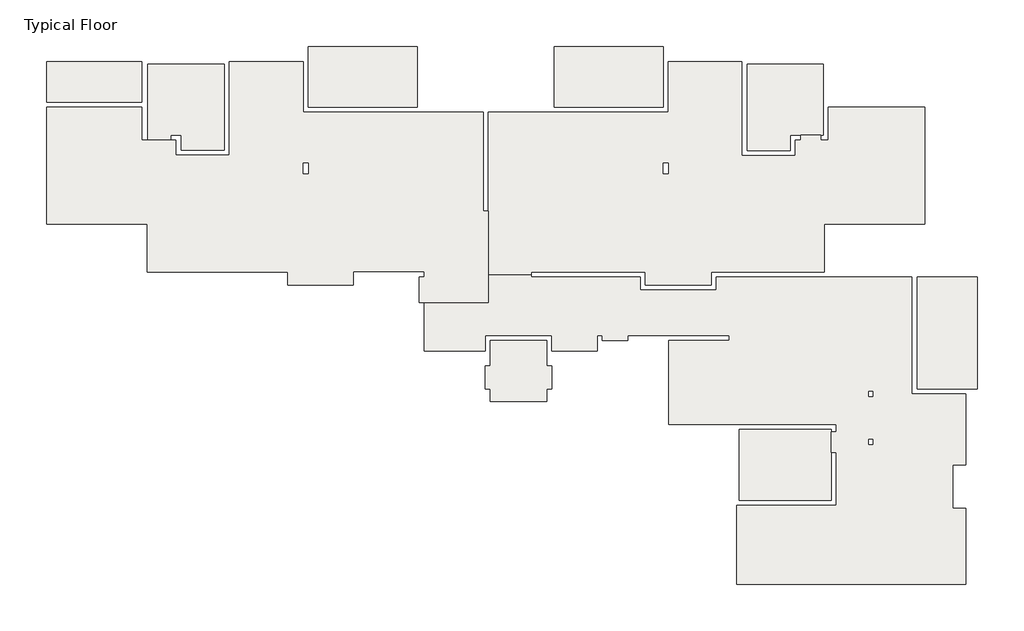
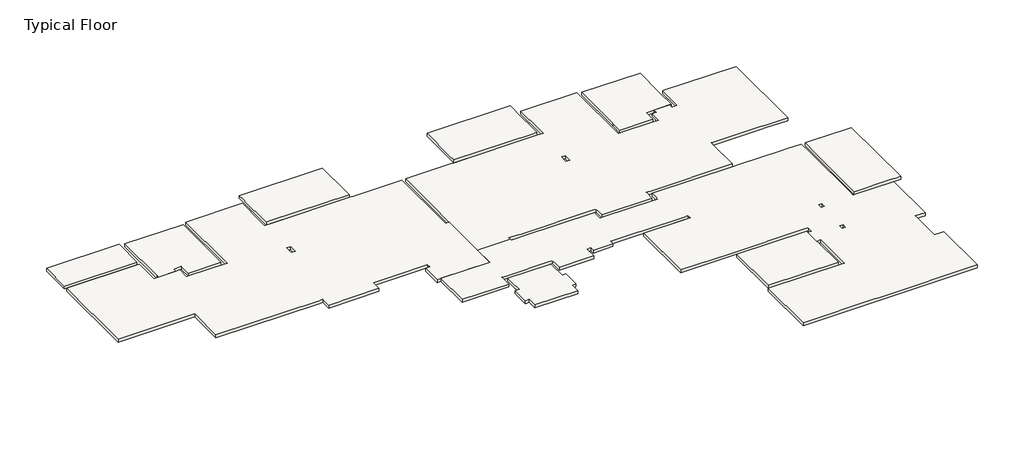
# One storey: 11 slabs.
"""IFC4 building model written with IfcOpenShell, lengths in millimetres."""

from ifc_helpers import new_model, si_unit, origin, place, context, project, spatial, faceted_brep, element, save

model = new_model("IFC4")

# Units and contexts
model_context = context("Model", 3, world=origin())
ifc_project = project(units=[si_unit("LENGTHUNIT", "METRE", prefix="MILLI")], contexts=[model_context])

# Site, building, storey
site = spatial("IfcSite", under=ifc_project)
building = spatial("IfcBuilding", under=site)
storey = spatial("IfcBuildingStorey", under=building, Name="Typical Floor", Elevation=3000.0)

# Slabs
placement = place(None, origin())
element("IfcSlab", 1, ObjectType="16", at=placement, inside=storey, context=model_context, shape_type="Brep", body=[
    faceted_brep([(21265.0782187, -24925.0312743, 2840.0), (21465.0782187, -24925.0312743, 2840.0), (21465.0782187, -24325.0312743, 2840.0), (21465.0782187, -23922.9713632, 2840.0), (23683.1266142, -23922.9713632, 2840.0), (23683.1266142, -24325.0312743, 2840.0), (23683.1266142, -24525.0312743, 2840.0), (23683.1266142, -24925.0312743, 2840.0), (23883.1266142, -24925.0312743, 2840.0), (23883.1266142, -25822.9713632, 2840.0), (23683.1266142, -25822.9713632, 2840.0), (23683.1266142, -26322.9713632, 2840.0), (21465.0782187, -26322.9713632, 2840.0), (21465.0782187, -25822.9713632, 2840.0), (21265.0782187, -25822.9713632, 2840.0), (21465.0782187, -24925.0312743, 3000.0), (21265.0782187, -24925.0312743, 3000.0), (21265.0782187, -25822.9713632, 3000.0), (21465.0782187, -25822.9713632, 3000.0), (21465.0782187, -26322.9713632, 3000.0), (23683.1266142, -26322.9713632, 3000.0), (23683.1266142, -25822.9713632, 3000.0), (23883.1266142, -25822.9713632, 3000.0), (23883.1266142, -24925.0312743, 3000.0), (23683.1266142, -24925.0312743, 3000.0), (23683.1266142, -24525.0312743, 3000.0), (23683.1266142, -24325.0312743, 3000.0), (23683.1266142, -23922.9713632, 3000.0), (21465.0782187, -23922.9713632, 3000.0), (21465.0782187, -24325.0312743, 3000.0), (23683.1266142, -26322.9713632, 2850.0), (21465.0782187, -26322.9713632, 2850.0)], [[[0, 1, 2, 3, 4, 5, 6, 7, 8, 9, 10, 11, 12, 13, 14]], [[15, 16, 17, 18, 19, 20, 21, 22, 23, 24, 25, 26, 27, 28, 29]], [[1, 0, 16, 15]], [[1, 15, 29, 28, 3, 2]], [[4, 3, 28, 27]], [[4, 27, 26, 25, 24, 7, 6, 5]], [[8, 7, 24, 23]], [[9, 8, 23, 22]], [[10, 9, 22, 21]], [[11, 10, 21, 20, 30]], [[12, 11, 30, 20, 19, 31]], [[13, 12, 31, 19, 18]], [[14, 13, 18, 17]], [[0, 14, 17, 16]]]),
])
element("IfcSlab", 2, ObjectType="16", at=placement, inside=storey, context=model_context, shape_type="Brep", body=[
    faceted_brep([(18665.0782187, -21404.9991523, 2840.0), (18865.0782187, -21404.9991523, 2840.0), (18865.0782187, -21204.9991523, 2840.0), (16065.0782187, -21204.9991523, 2840.0), (16065.0782187, -21404.9991523, 2840.0), (16065.0782187, -21724.9991523, 2840.0), (13465.4456872, -21724.9991523, 2840.0), (13465.4456872, -21417.3313694, 2840.0), (13465.4456872, -21217.3313694, 2840.0), (13265.4456872, -21217.3313694, 2840.0), (7932.8726521, -21217.3313694, 2840.0), (7932.8726521, -19524.5221497, 2840.0), (7932.8726521, -19324.5221497, 2840.0), (7532.8726521, -19324.5221497, 2840.0), (3964.5925114, -19324.5221497, 2840.0), (3964.5925114, -14717.2626845, 2840.0), (7711.7769333, -14717.2626845, 2840.0), (7711.7769333, -16016.1045626, 2840.0), (7961.7769333, -16016.1045626, 2840.0), (8856.7769333, -16016.1045626, 2840.0), (9066.7769333, -16016.1045626, 2840.0), (9066.7769333, -16605.3286465, 2840.0), (9266.7769333, -16605.3286465, 2840.0), (11166.7769333, -16605.3286465, 2840.0), (11166.7769333, -16405.3286465, 2840.0), (11166.7769333, -12916.1045626, 2840.0), (14076.6245949, -12916.1045626, 2840.0), (14076.6245949, -14515.7476445, 2840.0), (14076.6245949, -14915.7476445, 2840.0), (14476.6245949, -14915.7476445, 2840.0), (18576.6245949, -14915.7476445, 2840.0), (18576.6245949, -14917.2626845, 2840.0), (18776.6245949, -14917.2626845, 2840.0), (18776.6245949, -14915.7476445, 2840.0), (21178.4466499, -14915.7476445, 2840.0), (21178.4466499, -18413.3840407, 2840.0), (21178.4466499, -18813.3840407, 2840.0), (21378.4466499, -18813.3840407, 2840.0), (21378.4466499, -21325.0312743, 2840.0), (21378.4466499, -22425.0312743, 2840.0), (18865.0782187, -22425.0312743, 2840.0), (18665.0782187, -22425.0312743, 2840.0), (14276.6245949, -16922.7697624, 2840.0), (14076.6245949, -16922.7697624, 2840.0), (14076.6245949, -17322.7697624, 2840.0), (14276.6245949, -17322.7697624, 2840.0), (18865.0782187, -21404.9991523, 3000.0), (18665.0782187, -21404.9991523, 3000.0), (18665.0782187, -22425.0312743, 3000.0), (18865.0782187, -22425.0312743, 3000.0), (21378.4466499, -22425.0312743, 3000.0), (21378.4466499, -21325.0312743, 3000.0), (21378.4466499, -18813.3840407, 3000.0), (21178.4466499, -18813.3840407, 3000.0), (21178.4466499, -18413.3840407, 3000.0), (21178.4466499, -14915.7476445, 3000.0), (18776.6245949, -14915.7476445, 3000.0), (18776.6245949, -14917.2626845, 3000.0), (18576.6245949, -14917.2626845, 3000.0), (18576.6245949, -14915.7476445, 3000.0), (14476.6245949, -14915.7476445, 3000.0), (14076.6245949, -14915.7476445, 3000.0), (14076.6245949, -14515.7476445, 3000.0), (14076.6245949, -12916.1045626, 3000.0), (11166.7769333, -12916.1045626, 3000.0), (11166.7769333, -16405.3286465, 3000.0), (11166.7769333, -16605.3286465, 3000.0), (9266.7769333, -16605.3286465, 3000.0), (9066.7769333, -16605.3286465, 3000.0), (9066.7769333, -16016.1045626, 3000.0), (8856.7769333, -16016.1045626, 3000.0), (7961.7769333, -16016.1045626, 3000.0), (7711.7769333, -16016.1045626, 3000.0), (7711.7769333, -14717.2626845, 3000.0), (3964.5925114, -14717.2626845, 3000.0), (3964.5925114, -19324.5221497, 3000.0), (7532.8726521, -19324.5221497, 3000.0), (7932.8726521, -19324.5221497, 3000.0), (7932.8726521, -19524.5221497, 3000.0), (7932.8726521, -21217.3313694, 3000.0), (13265.4456872, -21217.3313694, 3000.0), (13465.4456872, -21217.3313694, 3000.0), (13465.4456872, -21417.3313694, 3000.0), (13465.4456872, -21724.9991523, 3000.0), (16065.0782187, -21724.9991523, 3000.0), (16065.0782187, -21404.9991523, 3000.0), (16065.0782187, -21204.9991523, 3000.0), (18865.0782187, -21204.9991523, 3000.0), (14076.6245949, -16922.7697624, 3000.0), (14276.6245949, -16922.7697624, 3000.0), (14276.6245949, -17322.7697624, 3000.0), (14076.6245949, -17322.7697624, 3000.0), (3964.5925114, -14717.2626845, 2850.0), (7711.7769333, -14717.2626845, 2850.0)], [[[0, 1, 2, 3, 4, 5, 6, 7, 8, 9, 10, 11, 12, 13, 14, 15, 16, 17, 18, 19, 20, 21, 22, 23, 24, 25, 26, 27, 28, 29, 30, 31, 32, 33, 34, 35, 36, 37, 38, 39, 40, 41], [42, 43, 44, 45]], [[46, 47, 48, 49, 50, 51, 52, 53, 54, 55, 56, 57, 58, 59, 60, 61, 62, 63, 64, 65, 66, 67, 68, 69, 70, 71, 72, 73, 74, 75, 76, 77, 78, 79, 80, 81, 82, 83, 84, 85, 86, 87], [88, 89, 90, 91]], [[1, 0, 47, 46]], [[2, 1, 46, 87]], [[3, 2, 87, 86]], [[3, 86, 85, 84, 5, 4]], [[6, 5, 84, 83]], [[6, 83, 82, 81, 8, 7]], [[8, 81, 80, 79, 10, 9]], [[10, 79, 78, 77, 12, 11]], [[12, 77, 76, 75, 14, 13]], [[15, 14, 75, 74, 92]], [[16, 15, 92, 74, 73, 93]], [[17, 16, 93, 73, 72]], [[18, 17, 72, 71]], [[18, 71, 70, 69, 20, 19]], [[21, 20, 69, 68]], [[21, 68, 67, 66, 23, 22]], [[23, 66, 65, 64, 25, 24]], [[26, 25, 64, 63]], [[26, 63, 62, 61, 28, 27]], [[55, 34, 33, 56]], [[28, 61, 60, 59, 30, 29]], [[34, 55, 54, 53, 36, 35]], [[37, 36, 53, 52]], [[39, 38, 37, 52, 51, 50]], [[41, 40, 39, 50, 49, 48]], [[0, 41, 48, 47]], [[43, 42, 89, 88]], [[44, 43, 88, 91]], [[45, 44, 91, 90]], [[42, 45, 90, 89]], [[32, 57, 56, 33]], [[57, 32, 31, 58]], [[58, 31, 30, 59]]]),
])
element("IfcSlab", 3, ObjectType="16", at=placement, inside=storey, context=model_context, shape_type="Brep", body=[
    faceted_brep([(7711.7769333, -12916.1045626, 2840.0), (7711.7769333, -14517.2626845, 2840.0), (3964.5925114, -14517.2626845, 2840.0), (3964.5925114, -12916.1045626, 2840.0), (7711.7769333, -14517.2626845, 3000.0), (7711.7769333, -13016.1045626, 3000.0), (7711.7769333, -12916.1045626, 3000.0), (3964.5925114, -12916.1045626, 3000.0), (3964.5925114, -14517.2626845, 3000.0), (7711.7769333, -14517.2626845, 2850.0), (3964.5925114, -14517.2626845, 2850.0), (3964.5925114, -12916.1045626, 2850.0)], [[[0, 1, 2, 3]], [[4, 5, 6, 7, 8]], [[1, 0, 6, 5, 4, 9]], [[2, 1, 9, 4, 8, 10]], [[3, 2, 10, 8, 7, 11]], [[0, 3, 11, 7, 6]]]),
])
element("IfcSlab", 4, ObjectType="16", at=placement, inside=storey, context=model_context, shape_type="Brep", body=[
    faceted_brep([(8856.7769333, -16016.1045626, 2840.0), (7961.7769333, -16016.1045626, 2840.0), (7961.7769333, -15916.1045626, 2840.0), (7961.7769333, -13016.1045626, 2840.0), (10966.7769333, -13016.1045626, 2840.0), (10966.7769333, -16405.3286465, 2840.0), (9266.7769333, -16405.3286465, 2840.0), (9266.7769333, -16016.1045626, 2840.0), (9266.7769333, -15816.1045626, 2840.0), (8856.7769333, -15816.1045626, 2840.0), (7961.7769333, -16016.1045626, 3000.0), (8856.7769333, -16016.1045626, 3000.0), (8856.7769333, -15816.1045626, 3000.0), (9266.7769333, -15816.1045626, 3000.0), (9266.7769333, -16016.1045626, 3000.0), (9266.7769333, -16405.3286465, 3000.0), (10966.7769333, -16405.3286465, 3000.0), (10966.7769333, -13016.1045626, 3000.0), (7961.7769333, -13016.1045626, 3000.0), (7961.7769333, -15916.1045626, 3000.0)], [[[0, 1, 2, 3, 4, 5, 6, 7, 8, 9]], [[10, 11, 12, 13, 14, 15, 16, 17, 18, 19]], [[1, 0, 11, 10]], [[2, 1, 10, 19]], [[3, 2, 19, 18]], [[4, 3, 18, 17]], [[5, 4, 17, 16]], [[6, 5, 16, 15]], [[6, 15, 14, 13, 8, 7]], [[9, 8, 13, 12]], [[0, 9, 12, 11]]]),
])
element("IfcSlab", 5, ObjectType="16", at=placement, inside=storey, context=model_context, shape_type="Brep", body=[
    faceted_brep([(18576.6245949, -12317.2626845, 2840.0), (18576.6245949, -14715.7476445, 2840.0), (14476.6245949, -14715.7476445, 2840.0), (14276.6245949, -14715.7476445, 2840.0), (14276.6245949, -14515.7476445, 2840.0), (14276.6245949, -12317.2626845, 2840.0), (18576.6245949, -14715.7476445, 3000.0), (18576.6245949, -14317.2626845, 3000.0), (18576.6245949, -12317.2626845, 3000.0), (14276.6245949, -12317.2626845, 3000.0), (14276.6245949, -12716.1045626, 3000.0), (14276.6245949, -12916.1045626, 3000.0), (14276.6245949, -14515.7476445, 3000.0), (14276.6245949, -14715.7476445, 3000.0), (14476.6245949, -14715.7476445, 3000.0)], [[[0, 1, 2, 3, 4, 5]], [[6, 7, 8, 9, 10, 11, 12, 13, 14]], [[1, 0, 8, 7, 6]], [[1, 6, 14, 13, 3, 2]], [[3, 13, 12, 11, 10, 9, 5, 4]], [[0, 5, 9, 8]]]),
])
element("IfcSlab", 6, ObjectType="16", at=placement, inside=storey, context=model_context, shape_type="Brep", body=[
    faceted_brep([(23984.4934221, -14715.7476445, 2840.0), (23984.4934221, -12317.2626845, 2840.0), (28282.0540099, -12317.2626845, 2840.0), (28282.0540099, -14515.7476445, 2840.0), (28282.0540099, -14715.7476445, 2840.0), (28082.0540099, -14715.7476445, 2840.0), (23984.4934221, -12317.2626845, 3000.0), (23984.4934221, -14317.2626845, 3000.0), (23984.4934221, -14715.7476445, 3000.0), (28082.0540099, -14715.7476445, 3000.0), (28282.0540099, -14715.7476445, 3000.0), (28282.0540099, -14515.7476445, 3000.0), (28282.0540099, -12916.1045626, 3000.0), (28282.0540099, -12716.1045626, 3000.0), (28282.0540099, -12317.2626845, 3000.0)], [[[0, 1, 2, 3, 4, 5]], [[6, 7, 8, 9, 10, 11, 12, 13, 14]], [[10, 4, 3, 2, 14, 13, 12, 11]], [[4, 10, 9, 8, 0, 5]], [[1, 0, 8, 7, 6]], [[2, 1, 6, 14]]]),
])
element("IfcSlab", 7, ObjectType="16", at=placement, inside=storey, context=model_context, shape_type="Brep", body=[
    faceted_brep([(34891.7617084, -27429.5129889, 2840.0), (34891.7617084, -27529.5129889, 2840.0), (34891.7617084, -28329.5129889, 2840.0), (34891.7617084, -30229.5129889, 2840.0), (31275.7730306, -30229.5129889, 2840.0), (31275.7730306, -27429.5129889, 2840.0), (34891.7617084, -27429.5129889, 3000.0), (31275.7730306, -27429.5129889, 3000.0), (31275.7730306, -30229.5129889, 3000.0), (34891.7617084, -30229.5129889, 3000.0), (34891.7617084, -28329.5129889, 3000.0), (34891.7617084, -27529.5129889, 3000.0)], [[[0, 1, 2, 3, 4, 5]], [[6, 7, 8, 9, 10, 11]], [[3, 2, 1, 0, 6, 11, 10, 9]], [[4, 3, 9, 8]], [[5, 4, 8, 7]], [[0, 5, 7, 6]]]),
])
element("IfcSlab", 8, ObjectType="16", at=placement, inside=storey, context=model_context, shape_type="Brep", body=[
    faceted_brep([(40664.8755666, -21417.3313694, 2840.0), (40664.8755666, -25825.2456589, 2840.0), (38283.1095165, -25825.2456589, 2840.0), (38283.1095165, -21417.3313694, 2840.0), (40664.8755666, -21417.3313694, 3000.0), (40184.8755666, -21417.3313694, 3000.0), (39784.8755666, -21417.3313694, 3000.0), (38283.1095165, -21417.3313694, 3000.0), (38283.1095165, -21967.4922699, 3000.0), (38283.1095165, -22167.4922699, 3000.0), (38283.1095165, -25825.2456589, 3000.0), (40196.0050664, -25825.2456589, 3000.0), (40396.0050664, -25825.2456589, 3000.0), (40664.8755666, -25825.2456589, 3000.0)], [[[0, 1, 2, 3]], [[4, 5, 6, 7, 8, 9, 10, 11, 12, 13]], [[1, 0, 4, 13]], [[2, 1, 13, 12, 11, 10]], [[3, 2, 10, 9, 8, 7]], [[0, 3, 7, 6, 5, 4]]]),
])
element("IfcSlab", 9, ObjectType="16", at=placement, inside=storey, context=model_context, shape_type="Brep", body=[
    faceted_brep([(31180.4949796, -30429.5129889, 2840.0), (35091.7617084, -30429.5129889, 2840.0), (35091.7617084, -30229.5129889, 2840.0), (35091.7617084, -28329.5129889, 2840.0), (34891.7617084, -28329.5129889, 2840.0), (34891.7617084, -27529.5129889, 2840.0), (35091.7617084, -27529.5129889, 2840.0), (35091.7617084, -27229.5129889, 2840.0), (34891.7617084, -27229.5129889, 2840.0), (30975.7730306, -27229.5129889, 2840.0), (28484.6380738, -27229.5129889, 2840.0), (28484.6380738, -23922.9713632, 2840.0), (30682.3560786, -23922.9713632, 2840.0), (30882.3560786, -23922.9713632, 2840.0), (30882.3560786, -23722.9713632, 2840.0), (30682.3560786, -23722.9713632, 2840.0), (28484.6380738, -23722.9713632, 2840.0), (28284.6380738, -23722.9713632, 2840.0), (26884.6380738, -23722.9713632, 2840.0), (26884.6380738, -23922.9713632, 2840.0), (25866.8915333, -23922.9713632, 2840.0), (25866.8915333, -23725.0312743, 2840.0), (25666.8915333, -23725.0312743, 2840.0), (25666.8915333, -24325.0312743, 2840.0), (23883.1266142, -24325.0312743, 2840.0), (23883.1266142, -23922.9713632, 2840.0), (23883.1266142, -23722.9713632, 2840.0), (23683.1266142, -23722.9713632, 2840.0), (21465.0782187, -23722.9713632, 2840.0), (21265.0782187, -23722.9713632, 2840.0), (21265.0782187, -23922.9713632, 2840.0), (21265.0782187, -24325.0312743, 2840.0), (18865.0782187, -24325.0312743, 2840.0), (18865.0782187, -22425.0312743, 2840.0), (21378.4466499, -22425.0312743, 2840.0), (21378.4466499, -21325.0312743, 2840.0), (23078.0627315, -21325.0312743, 2840.0), (23078.0627315, -21417.3313694, 2840.0), (23478.0627315, -21417.3313694, 2840.0), (23678.0627315, -21417.3313694, 2840.0), (27376.8445171, -21417.3313694, 2840.0), (27376.8445171, -21924.9991523, 2840.0), (27576.8445171, -21924.9991523, 2840.0), (30175.7089043, -21924.9991523, 2840.0), (30375.7089043, -21924.9991523, 2840.0), (30375.7089043, -21724.9991523, 2840.0), (30375.7089043, -21417.3313694, 2840.0), (34621.395755, -21417.3313694, 2840.0), (34821.395755, -21417.3313694, 2840.0), (37118.3892225, -21417.3313694, 2840.0), (37318.3892225, -21417.3313694, 2840.0), (38083.1095165, -21417.3313694, 2840.0), (38083.1095165, -21967.4922699, 2840.0), (38083.1095165, -22167.4922699, 2840.0), (38083.1095165, -25825.2456589, 2840.0), (38083.1095165, -26025.2456589, 2840.0), (38283.1095165, -26025.2456589, 2840.0), (40196.0050664, -26025.2456589, 2840.0), (40196.0050664, -28831.9248672, 2840.0), (39694.7023527, -28831.9248672, 2840.0), (39694.7023527, -29031.9248672, 2840.0), (39696.0050664, -29031.9248672, 2840.0), (39696.0050664, -30330.1793317, 2840.0), (39696.0050664, -30530.1793317, 2840.0), (40196.0050664, -30530.1793317, 2840.0), (40196.0050664, -33427.8618321, 2840.0), (40196.0050664, -33527.8618321, 2840.0), (40096.0050664, -33527.8618321, 2840.0), (31180.4949796, -33527.8618321, 2840.0), (36543.2842271, -26125.0806557, 2840.0), (36543.2842271, -25925.0806557, 2840.0), (36383.2842271, -25925.0806557, 2840.0), (36383.2842271, -26125.0806557, 2840.0), (36543.2842271, -28019.1243939, 2840.0), (36543.2842271, -27819.1243939, 2840.0), (36383.2842271, -27819.1243939, 2840.0), (36383.2842271, -28019.1243939, 2840.0), (35091.7617084, -30429.5129889, 3000.0), (31180.4949796, -30429.5129889, 3000.0), (31180.4949796, -33527.8618321, 3000.0), (34886.984967, -33527.8618321, 3000.0), (35086.984967, -33527.8618321, 3000.0), (37584.3945148, -33527.8618321, 3000.0), (37784.3945148, -33527.8618321, 3000.0), (40096.0050664, -33527.8618321, 3000.0), (40196.0050664, -33527.8618321, 3000.0), (40196.0050664, -33427.8618321, 3000.0), (40196.0050664, -30530.1793317, 3000.0), (39696.0050664, -30530.1793317, 3000.0), (39696.0050664, -30330.1793317, 3000.0), (39696.0050664, -29031.9248672, 3000.0), (39694.7023527, -29031.9248672, 3000.0), (39694.7023527, -28831.9248672, 3000.0), (40196.0050664, -28831.9248672, 3000.0), (40196.0050664, -26025.2456589, 3000.0), (38283.1095165, -26025.2456589, 3000.0), (38083.1095165, -26025.2456589, 3000.0), (38083.1095165, -25825.2456589, 3000.0), (38083.1095165, -22167.4922699, 3000.0), (38083.1095165, -21967.4922699, 3000.0), (38083.1095165, -21417.3313694, 3000.0), (37318.3892225, -21417.3313694, 3000.0), (37118.3892225, -21417.3313694, 3000.0), (34821.395755, -21417.3313694, 3000.0), (34621.395755, -21417.3313694, 3000.0), (30375.7089043, -21417.3313694, 3000.0), (30375.7089043, -21724.9991523, 3000.0), (30375.7089043, -21924.9991523, 3000.0), (30175.7089043, -21924.9991523, 3000.0), (27576.8445171, -21924.9991523, 3000.0), (27376.8445171, -21924.9991523, 3000.0), (27376.8445171, -21417.3313694, 3000.0), (23678.0627315, -21417.3313694, 3000.0), (23478.0627315, -21417.3313694, 3000.0), (23078.0627315, -21417.3313694, 3000.0), (23078.0627315, -21325.0312743, 3000.0), (21378.4466499, -21325.0312743, 3000.0), (21378.4466499, -22425.0312743, 3000.0), (18865.0782187, -22425.0312743, 3000.0), (18865.0782187, -24325.0312743, 3000.0), (21265.0782187, -24325.0312743, 3000.0), (21265.0782187, -23922.9713632, 3000.0), (21265.0782187, -23722.9713632, 3000.0), (21465.0782187, -23722.9713632, 3000.0), (23683.1266142, -23722.9713632, 3000.0), (23883.1266142, -23722.9713632, 3000.0), (23883.1266142, -23922.9713632, 3000.0), (23883.1266142, -24325.0312743, 3000.0), (25666.8915333, -24325.0312743, 3000.0), (25666.8915333, -23725.0312743, 3000.0), (25866.8915333, -23725.0312743, 3000.0), (25866.8915333, -23922.9713632, 3000.0), (26884.6380738, -23922.9713632, 3000.0), (26884.6380738, -23722.9713632, 3000.0), (28284.6380738, -23722.9713632, 3000.0), (28484.6380738, -23722.9713632, 3000.0), (30682.3560786, -23722.9713632, 3000.0), (30882.3560786, -23722.9713632, 3000.0), (30882.3560786, -23922.9713632, 3000.0), (30682.3560786, -23922.9713632, 3000.0), (28484.6380738, -23922.9713632, 3000.0), (28484.6380738, -27229.5129889, 3000.0), (30975.7730306, -27229.5129889, 3000.0), (34891.7617084, -27229.5129889, 3000.0), (35091.7617084, -27229.5129889, 3000.0), (35091.7617084, -27529.5129889, 3000.0), (34891.7617084, -27529.5129889, 3000.0), (34891.7617084, -28329.5129889, 3000.0), (35091.7617084, -28329.5129889, 3000.0), (35091.7617084, -30229.5129889, 3000.0), (36543.2842271, -25925.0806557, 3000.0), (36543.2842271, -26125.0806557, 3000.0), (36383.2842271, -26125.0806557, 3000.0), (36383.2842271, -25925.0806557, 3000.0), (36543.2842271, -27819.1243939, 3000.0), (36543.2842271, -28019.1243939, 3000.0), (36383.2842271, -28019.1243939, 3000.0), (36383.2842271, -27819.1243939, 3000.0), (39696.0050664, -29031.9248672, 2850.0)], [[[0, 1, 2, 3, 4, 5, 6, 7, 8, 9, 10, 11, 12, 13, 14, 15, 16, 17, 18, 19, 20, 21, 22, 23, 24, 25, 26, 27, 28, 29, 30, 31, 32, 33, 34, 35, 36, 37, 38, 39, 40, 41, 42, 43, 44, 45, 46, 47, 48, 49, 50, 51, 52, 53, 54, 55, 56, 57, 58, 59, 60, 61, 62, 63, 64, 65, 66, 67, 68], [69, 70, 71, 72], [73, 74, 75, 76]], [[77, 78, 79, 80, 81, 82, 83, 84, 85, 86, 87, 88, 89, 90, 91, 92, 93, 94, 95, 96, 97, 98, 99, 100, 101, 102, 103, 104, 105, 106, 107, 108, 109, 110, 111, 112, 113, 114, 115, 116, 117, 118, 119, 120, 121, 122, 123, 124, 125, 126, 127, 128, 129, 130, 131, 132, 133, 134, 135, 136, 137, 138, 139, 140, 141, 142, 143, 144, 145, 146, 147, 148, 149], [150, 151, 152, 153], [154, 155, 156, 157]], [[1, 0, 78, 77]], [[1, 77, 149, 148, 3, 2]], [[4, 3, 148, 147]], [[5, 4, 147, 146]], [[6, 5, 146, 145]], [[7, 6, 145, 144]], [[7, 144, 143, 142, 141, 10, 9, 8]], [[11, 10, 141, 140]], [[11, 140, 139, 138, 13, 12]], [[14, 13, 138, 137]], [[14, 137, 136, 135, 134, 133, 18, 17, 16, 15]], [[19, 18, 133, 132]], [[20, 19, 132, 131]], [[21, 20, 131, 130]], [[22, 21, 130, 129]], [[23, 22, 129, 128]], [[24, 23, 128, 127]], [[24, 127, 126, 125, 26, 25]], [[26, 125, 124, 123, 122, 29, 28, 27]], [[29, 122, 121, 120, 31, 30]], [[32, 31, 120, 119]], [[33, 32, 119, 118]], [[34, 33, 118, 117]], [[35, 34, 117, 116]], [[36, 35, 116, 115]], [[37, 36, 115, 114]], [[37, 114, 113, 112, 111, 40, 39, 38]], [[41, 40, 111, 110]], [[41, 110, 109, 108, 107, 44, 43, 42]], [[44, 107, 106, 105, 46, 45]], [[46, 105, 104, 103, 102, 101, 100, 51, 50, 49, 48, 47]], [[51, 100, 99, 98, 97, 96, 55, 54, 53, 52]], [[55, 96, 95, 94, 57, 56]], [[58, 57, 94, 93]], [[58, 93, 92, 59]], [[88, 63, 62, 61, 158, 90, 89]], [[64, 63, 88, 87]], [[64, 87, 86, 85, 66, 65]], [[66, 85, 84, 83, 82, 81, 80, 79, 68, 67]], [[0, 68, 79, 78]], [[60, 91, 90, 158, 61]], [[59, 92, 91, 60]], [[69, 151, 150, 70]], [[151, 69, 72, 152]], [[152, 72, 71, 153]], [[153, 71, 70, 150]], [[73, 155, 154, 74]], [[155, 73, 76, 156]], [[156, 76, 75, 157]], [[157, 75, 74, 154]]]),
])
element("IfcSlab", 10, ObjectType="16", at=placement, inside=storey, context=model_context, shape_type="Brep", body=[
    faceted_brep([(28482.0540099, -12916.1045626, 2840.0), (31380.8167217, -12916.1045626, 2840.0), (31380.8167217, -16617.2626845, 2840.0), (31580.8167217, -16617.2626845, 2840.0), (33290.8167217, -16617.2626845, 2840.0), (33490.8167217, -16617.2626845, 2840.0), (33490.8167217, -16017.2626845, 2840.0), (33690.8167217, -16017.2626845, 2840.0), (33690.8167217, -15817.2626845, 2840.0), (34490.8167217, -15817.2626845, 2840.0), (34490.8167217, -16017.2626845, 2840.0), (34790.8167217, -16017.2626845, 2840.0), (34790.8167217, -15817.2626845, 2840.0), (34790.8167217, -14717.2626845, 2840.0), (34840.8167217, -14717.2626845, 2840.0), (38480.9633489, -14717.2626845, 2840.0), (38580.9633489, -14717.2626845, 2840.0), (38580.9633489, -14817.2626845, 2840.0), (38580.9633489, -19324.5221497, 2840.0), (37421.6505657, -19324.5221497, 2840.0), (37221.6505657, -19324.5221497, 2840.0), (34821.395755, -19324.5221497, 2840.0), (34621.395755, -19324.5221497, 2840.0), (34621.395755, -19524.5221497, 2840.0), (34621.395755, -21217.3313694, 2840.0), (30375.7089043, -21217.3313694, 2840.0), (30175.7089043, -21217.3313694, 2840.0), (30175.7089043, -21724.9991523, 2840.0), (27576.8445171, -21724.9991523, 2840.0), (27576.8445171, -21417.3313694, 2840.0), (27576.8445171, -21217.3313694, 2840.0), (27376.8445171, -21217.3313694, 2840.0), (23678.0627315, -21217.3313694, 2840.0), (23478.0627315, -21217.3313694, 2840.0), (23078.0627315, -21217.3313694, 2840.0), (23078.0627315, -21325.0312743, 2840.0), (21378.4466499, -21325.0312743, 2840.0), (21378.4466499, -18813.3840407, 2840.0), (21378.4466499, -18413.3840407, 2840.0), (21378.4466499, -14915.7476445, 2840.0), (21380.7780067, -14915.7476445, 2840.0), (21780.7780067, -14915.7476445, 2840.0), (23784.4934221, -14915.7476445, 2840.0), (23784.4934221, -14917.2626845, 2840.0), (23984.4934221, -14917.2626845, 2840.0), (23984.4934221, -14915.7476445, 2840.0), (28082.0540099, -14915.7476445, 2840.0), (28482.0540099, -14915.7476445, 2840.0), (28482.0540099, -14515.7476445, 2840.0), (28476.6245949, -17322.7697624, 2840.0), (28476.6245949, -16922.7697624, 2840.0), (28276.6245949, -16922.7697624, 2840.0), (28276.6245949, -17322.7697624, 2840.0), (31380.8167217, -12916.1045626, 3000.0), (28482.0540099, -12916.1045626, 3000.0), (28482.0540099, -14515.7476445, 3000.0), (28482.0540099, -14915.7476445, 3000.0), (28082.0540099, -14915.7476445, 3000.0), (23984.4934221, -14915.7476445, 3000.0), (23984.4934221, -14917.2626845, 3000.0), (23784.4934221, -14917.2626845, 3000.0), (23784.4934221, -14915.7476445, 3000.0), (21780.7780067, -14915.7476445, 3000.0), (21380.7780067, -14915.7476445, 3000.0), (21378.4466499, -14915.7476445, 3000.0), (21378.4466499, -18413.3840407, 3000.0), (21378.4466499, -18813.3840407, 3000.0), (21378.4466499, -21325.0312743, 3000.0), (23078.0627315, -21325.0312743, 3000.0), (23078.0627315, -21217.3313694, 3000.0), (23478.0627315, -21217.3313694, 3000.0), (23678.0627315, -21217.3313694, 3000.0), (27376.8445171, -21217.3313694, 3000.0), (27576.8445171, -21217.3313694, 3000.0), (27576.8445171, -21417.3313694, 3000.0), (27576.8445171, -21724.9991523, 3000.0), (30175.7089043, -21724.9991523, 3000.0), (30175.7089043, -21217.3313694, 3000.0), (30375.7089043, -21217.3313694, 3000.0), (34621.395755, -21217.3313694, 3000.0), (34621.395755, -19524.5221497, 3000.0), (34621.395755, -19324.5221497, 3000.0), (34821.395755, -19324.5221497, 3000.0), (37221.6505657, -19324.5221497, 3000.0), (37421.6505657, -19324.5221497, 3000.0), (38580.9633489, -19324.5221497, 3000.0), (38580.9633489, -14817.2626845, 3000.0), (38580.9633489, -14717.2626845, 3000.0), (38480.9633489, -14717.2626845, 3000.0), (34840.8167217, -14717.2626845, 3000.0), (34790.8167217, -14717.2626845, 3000.0), (34790.8167217, -15817.2626845, 3000.0), (34790.8167217, -16017.2626845, 3000.0), (34490.8167217, -16017.2626845, 3000.0), (34490.8167217, -15817.2626845, 3000.0), (33690.8167217, -15817.2626845, 3000.0), (33690.8167217, -16017.2626845, 3000.0), (33490.8167217, -16017.2626845, 3000.0), (33490.8167217, -16617.2626845, 3000.0), (33290.8167217, -16617.2626845, 3000.0), (31580.8167217, -16617.2626845, 3000.0), (31380.8167217, -16617.2626845, 3000.0), (28476.6245949, -16922.7697624, 3000.0), (28476.6245949, -17322.7697624, 3000.0), (28276.6245949, -17322.7697624, 3000.0), (28276.6245949, -16922.7697624, 3000.0), (38580.9633489, -19324.5221497, 2850.0)], [[[0, 1, 2, 3, 4, 5, 6, 7, 8, 9, 10, 11, 12, 13, 14, 15, 16, 17, 18, 19, 20, 21, 22, 23, 24, 25, 26, 27, 28, 29, 30, 31, 32, 33, 34, 35, 36, 37, 38, 39, 40, 41, 42, 43, 44, 45, 46, 47, 48], [49, 50, 51, 52]], [[53, 54, 55, 56, 57, 58, 59, 60, 61, 62, 63, 64, 65, 66, 67, 68, 69, 70, 71, 72, 73, 74, 75, 76, 77, 78, 79, 80, 81, 82, 83, 84, 85, 86, 87, 88, 89, 90, 91, 92, 93, 94, 95, 96, 97, 98, 99, 100, 101], [102, 103, 104, 105]], [[39, 64, 63, 62, 61, 42, 41, 40]], [[56, 47, 46, 45, 58, 57]], [[47, 56, 55, 54, 0, 48]], [[1, 0, 54, 53]], [[2, 1, 53, 101]], [[2, 101, 100, 99, 98, 5, 4, 3]], [[6, 5, 98, 97]], [[7, 6, 97, 96]], [[8, 7, 96, 95]], [[9, 8, 95, 94]], [[10, 9, 94, 93]], [[11, 10, 93, 92]], [[11, 92, 91, 90, 13, 12]], [[13, 90, 89, 88, 87, 16, 15, 14]], [[16, 87, 86, 85, 106, 18, 17]], [[18, 106, 85, 84, 83, 82, 81, 22, 21, 20, 19]], [[22, 81, 80, 79, 24, 23]], [[26, 25, 24, 79, 78, 77]], [[27, 26, 77, 76]], [[28, 27, 76, 75]], [[28, 75, 74, 73, 30, 29]], [[30, 73, 72, 71, 70, 69, 34, 33, 32, 31]], [[35, 34, 69, 68]], [[36, 35, 68, 67]], [[39, 38, 37, 36, 67, 66, 65, 64]], [[44, 59, 58, 45]], [[59, 44, 43, 60]], [[60, 43, 42, 61]], [[49, 103, 102, 50]], [[103, 49, 52, 104]], [[104, 52, 51, 105]], [[105, 51, 50, 102]]]),
])
element("IfcSlab", 11, ObjectType="16", at=placement, inside=storey, context=model_context, shape_type="Brep", body=[
    faceted_brep([(31580.8167217, -13016.1045626, 2840.0), (34590.8167217, -13016.1045626, 2840.0), (34590.8167217, -15817.2626845, 2840.0), (34490.8167217, -15817.2626845, 2840.0), (33690.8167217, -15817.2626845, 2840.0), (33290.8167217, -15817.2626845, 2840.0), (33290.8167217, -16017.2626845, 2840.0), (33290.8167217, -16417.2626845, 2840.0), (31580.8167217, -16417.2626845, 2840.0), (31580.8167217, -15817.2626845, 2840.0), (34590.8167217, -13016.1045626, 3000.0), (31580.8167217, -13016.1045626, 3000.0), (31580.8167217, -15817.2626845, 3000.0), (31580.8167217, -16417.2626845, 3000.0), (33290.8167217, -16417.2626845, 3000.0), (33290.8167217, -16017.2626845, 3000.0), (33290.8167217, -15817.2626845, 3000.0), (33690.8167217, -15817.2626845, 3000.0), (34490.8167217, -15817.2626845, 3000.0), (34590.8167217, -15817.2626845, 3000.0), (34590.8167217, -14717.2626845, 3000.0)], [[[0, 1, 2, 3, 4, 5, 6, 7, 8, 9]], [[10, 11, 12, 13, 14, 15, 16, 17, 18, 19, 20]], [[1, 0, 11, 10]], [[2, 1, 10, 20, 19]], [[2, 19, 18, 17, 16, 5, 4, 3]], [[5, 16, 15, 14, 7, 6]], [[8, 7, 14, 13]], [[9, 8, 13, 12]], [[0, 9, 12, 11]]]),
])

save(model, "model.ifc")

# Revit data of these elements
# Type "16"
#   Function = 0
#   Layers, outside or top first: 16 cm "Concrete" (function 1)
# Element 1 (IfcSlab, "16")
#   Mark = "S1"
#   SOFiSTiK_AMG_Comments = ""
#   built-in parameter 1001955 = 1.5708 (stored number, unit not read)
#   Height Offset From Level = 0 cm
#   built-in parameter 1001954 = 1
#   SOFiSTiK_AMG_Scheduled = yes
#   SOFiSTiK_AMG_Adjusted = yes
#   Phase Created = New Construction
#   Materials on its faces: "Concrete"
# Element 2 (IfcSlab, "16")
#   Mark = "S2"
#   SOFiSTiK_AMG_Comments = ""
#   built-in parameter 1001955 = 1.5708 (stored number, unit not read)
#   Height Offset From Level = 0 cm
#   built-in parameter 1001954 = 1
#   SOFiSTiK_AMG_Scheduled = yes
#   SOFiSTiK_AMG_Adjusted = yes
#   Phase Created = New Construction
#   Materials on its faces: "Concrete"
# Element 3 (IfcSlab, "16")
#   Mark = "S3"
#   SOFiSTiK_AMG_Comments = ""
#   Height Offset From Level = 0 cm
#   built-in parameter 1001954 = 1
#   SOFiSTiK_AMG_Scheduled = yes
#   SOFiSTiK_AMG_Adjusted = yes
#   Phase Created = New Construction
#   Materials on its faces: "Concrete"
# Element 4 (IfcSlab, "16")
#   Mark = "S4"
#   SOFiSTiK_AMG_Comments = ""
#   Height Offset From Level = 0 cm
#   built-in parameter 1001954 = 1
#   SOFiSTiK_AMG_Scheduled = yes
#   SOFiSTiK_AMG_Adjusted = yes
#   Phase Created = New Construction
#   Materials on its faces: "Concrete"
# Element 5 (IfcSlab, "16")
#   Mark = "S5"
#   SOFiSTiK_AMG_Comments = ""
#   Height Offset From Level = 0 cm
#   built-in parameter 1001954 = 1
#   SOFiSTiK_AMG_Scheduled = yes
#   SOFiSTiK_AMG_Adjusted = yes
#   Phase Created = New Construction
#   Materials on its faces: "Concrete"
# Element 6 (IfcSlab, "16")
#   Mark = "S6"
#   SOFiSTiK_AMG_Comments = ""
#   Height Offset From Level = 0 cm
#   built-in parameter 1001954 = 1
#   SOFiSTiK_AMG_Scheduled = yes
#   SOFiSTiK_AMG_Adjusted = yes
#   Phase Created = New Construction
#   Materials on its faces: "Concrete"
# Element 7 (IfcSlab, "16")
#   Mark = "S7"
#   SOFiSTiK_AMG_Comments = ""
#   Height Offset From Level = 0 cm
#   built-in parameter 1001954 = 1
#   SOFiSTiK_AMG_Scheduled = yes
#   SOFiSTiK_AMG_Adjusted = yes
#   Phase Created = New Construction
#   Materials on its faces: "Concrete"
# Element 8 (IfcSlab, "16")
#   Mark = "S8"
#   SOFiSTiK_AMG_Comments = ""
#   Height Offset From Level = 0 cm
#   built-in parameter 1001954 = 1
#   SOFiSTiK_AMG_Scheduled = yes
#   SOFiSTiK_AMG_Adjusted = yes
#   Phase Created = New Construction
#   Materials on its faces: "Concrete"
# Element 9 (IfcSlab, "16")
#   Mark = "S9"
#   SOFiSTiK_AMG_Comments = ""
#   built-in parameter 1001955 = 1.5708 (stored number, unit not read)
#   Height Offset From Level = 0 cm
#   built-in parameter 1001954 = 1
#   SOFiSTiK_AMG_Scheduled = yes
#   SOFiSTiK_AMG_Adjusted = yes
#   Phase Created = New Construction
#   Materials on its faces: "Concrete"
# Element 10 (IfcSlab, "16")
#   Mark = "S10"
#   SOFiSTiK_AMG_Comments = ""
#   built-in parameter 1001955 = 1.5708 (stored number, unit not read)
#   Height Offset From Level = 0 cm
#   built-in parameter 1001954 = 1
#   SOFiSTiK_AMG_Scheduled = yes
#   SOFiSTiK_AMG_Adjusted = yes
#   Phase Created = New Construction
#   Materials on its faces: "Concrete"
# Element 11 (IfcSlab, "16")
#   Mark = "S11"
#   SOFiSTiK_AMG_Comments = ""
#   built-in parameter 1001955 = 3.14159 (stored number, unit not read)
#   Height Offset From Level = 0 cm
#   built-in parameter 1001954 = 1
#   SOFiSTiK_AMG_Scheduled = yes
#   SOFiSTiK_AMG_Adjusted = yes
#   Phase Created = New Construction
#   Materials on its faces: "Concrete"
# Materials
#   "Concrete": class "Concrete", colour RGB 192 192 192, transparency 0, Keynote = "01000", Description = "Cast-in-place concrete", Cost = 0
